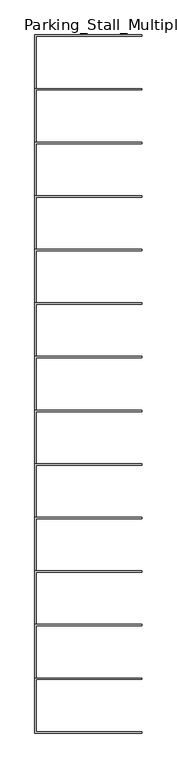
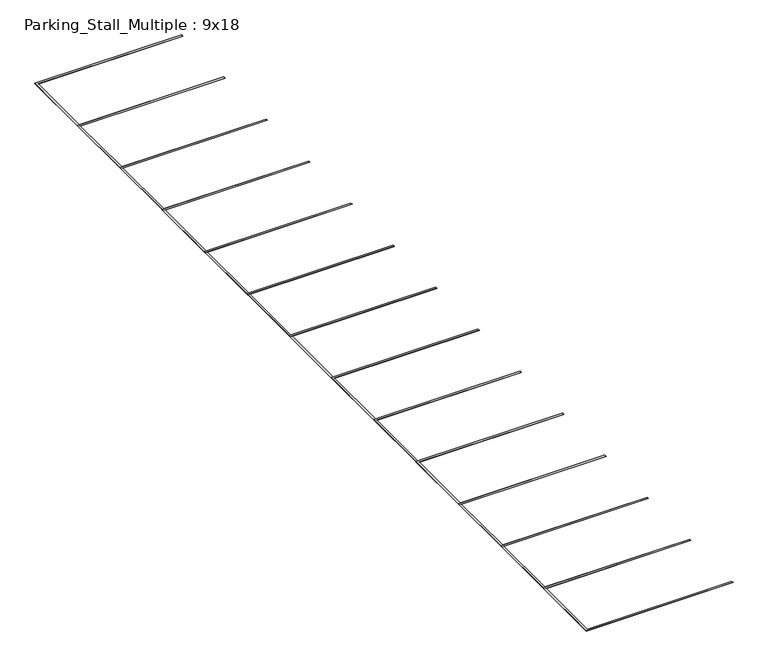
"""IFC4 building model written with IfcOpenShell, lengths in millimetres: proxy geometry, Parking_Stall_Multiple : 9x18."""

from ifc_helpers import new_model, si_unit, origin, origin_with_axes, place, context, project, spatial, polyline, outline, extrude, source, transform, mapped, element, save


def parking_stall_multiple_9x18_eccd42c3(model_context):
    return source(origin(), model_context, "Body", "SweptSolid", [
        extrude(outline(polyline([(5486.4, -32918.4), (5486.4, -32994.6), (76.2, -32994.6), (76.2, -35661.6), (5486.4, -35661.6), (5486.4, -35737.8), (0.0, -35737.8), (0.0, -32918.4), (5486.4, -32918.4)])), origin_with_axes(), (0.0, 0.0, 1.0), 6.35),
        extrude(outline(polyline([(5486.4, -30175.2), (5486.4, -30251.4), (76.2, -30251.4), (76.2, -32918.4), (5486.4, -32918.4), (5486.4, -32994.6), (0.0, -32994.6), (0.0, -30175.2), (5486.4, -30175.2)])), origin_with_axes(), (0.0, 0.0, 1.0), 6.35),
        extrude(outline(polyline([(5486.4, -27432.0), (5486.4, -27508.2), (76.2, -27508.2), (76.2, -30175.2), (5486.4, -30175.2), (5486.4, -30251.4), (0.0, -30251.4), (0.0, -27432.0), (5486.4, -27432.0)])), origin_with_axes(), (0.0, 0.0, 1.0), 6.35),
        extrude(outline(polyline([(5486.4, -24688.8), (5486.4, -24765.0), (76.2, -24765.0), (76.2, -27432.0), (5486.4, -27432.0), (5486.4, -27508.2), (0.0, -27508.2), (0.0, -24688.8), (5486.4, -24688.8)])), origin_with_axes(), (0.0, 0.0, 1.0), 6.35),
        extrude(outline(polyline([(5486.4, -21945.6), (5486.4, -22021.8), (76.2, -22021.8), (76.2, -24688.8), (5486.4, -24688.8), (5486.4, -24765.0), (0.0, -24765.0), (0.0, -21945.6), (5486.4, -21945.6)])), origin_with_axes(), (0.0, 0.0, 1.0), 6.35),
        extrude(outline(polyline([(5486.4, -19202.4), (5486.4, -19278.6), (76.2, -19278.6), (76.2, -21945.6), (5486.4, -21945.6), (5486.4, -22021.8), (0.0, -22021.8), (0.0, -19202.4), (5486.4, -19202.4)])), origin_with_axes(), (0.0, 0.0, 1.0), 6.35),
        extrude(outline(polyline([(5486.4, -16459.2), (5486.4, -16535.4), (76.2, -16535.4), (76.2, -19202.4), (5486.4, -19202.4), (5486.4, -19278.6), (0.0, -19278.6), (0.0, -16459.2), (5486.4, -16459.2)])), origin_with_axes(), (0.0, 0.0, 1.0), 6.35),
        extrude(outline(polyline([(5486.4, -13716.0), (5486.4, -13792.2), (76.2, -13792.2), (76.2, -16459.2), (5486.4, -16459.2), (5486.4, -16535.4), (0.0, -16535.4), (0.0, -13716.0), (5486.4, -13716.0)])), origin_with_axes(), (0.0, 0.0, 1.0), 6.35),
        extrude(outline(polyline([(5486.4, -10972.8), (5486.4, -11049.0), (76.2, -11049.0), (76.2, -13716.0), (5486.4, -13716.0), (5486.4, -13792.2), (0.0, -13792.2), (0.0, -10972.8), (5486.4, -10972.8)])), origin_with_axes(), (0.0, 0.0, 1.0), 6.35),
        extrude(outline(polyline([(5486.4, -8229.6), (5486.4, -8305.8), (76.2, -8305.8), (76.2, -10972.8), (5486.4, -10972.8), (5486.4, -11049.0), (0.0, -11049.0), (0.0, -8229.6), (5486.4, -8229.6)])), origin_with_axes(), (0.0, 0.0, 1.0), 6.35),
        extrude(outline(polyline([(5486.4, -5486.4), (5486.4, -5562.6), (76.2, -5562.6), (76.2, -8229.6), (5486.4, -8229.6), (5486.4, -8305.8), (0.0, -8305.8), (0.0, -5486.4), (5486.4, -5486.4)])), origin_with_axes(), (0.0, 0.0, 1.0), 6.35),
        extrude(outline(polyline([(5486.4, -2743.2), (5486.4, -2819.4), (76.2, -2819.4), (76.2, -5486.4), (5486.4, -5486.4), (5486.4, -5562.6), (0.0, -5562.6), (0.0, -2743.2), (5486.4, -2743.2)])), origin_with_axes(), (0.0, 0.0, 1.0), 6.35),
        extrude(outline(polyline([(5486.4, 0.0), (5486.4, -76.2), (76.2, -76.2), (76.2, -2743.2), (5486.4, -2743.2), (5486.4, -2819.4), (0.0, -2819.4), (0.0, 0.0), (5486.4, 0.0)])), origin_with_axes(), (0.0, 0.0, 1.0), 6.35),
    ])


if __name__ == "__main__":
    model = new_model("IFC4")
    model_context = context("Model", 3, world=origin())
    ifc_project = project(units=[si_unit("LENGTHUNIT", "METRE", prefix="MILLI")], contexts=[model_context])
    site = spatial("IfcSite", under=ifc_project)
    building = spatial("IfcBuilding", under=site)
    placement = place(None, origin())
    parking_stall_multiple_9x18_shape = parking_stall_multiple_9x18_eccd42c3(model_context)
    element("IfcBuildingElementProxy", 1, Name="Parking_Stall_Multiple : 9x18", ObjectType="Parking_Stall_Multiple : 9x18", at=placement, inside=building, context=model_context, shape_type="MappedRepresentation", body=[
        mapped(parking_stall_multiple_9x18_shape, transform((0.0, 0.0, 0.0), x_axis=(1.0, 0.0, 0.0), y_axis=(0.0, 1.0, 0.0), z_axis=(0.0, 0.0, 1.0))),
    ])
    save(model, "model.ifc")

# Revit data of these elements
# Type "Parking_Stall_Multiple : 9x18"
#   Parking_Width_M = 9' - 0"
#   Parking_Run_Length [instance default] = 65' - 0"
#   Parking_Line_Width = 0' - 3"
#   Parking_Length_M = 18' - 0"
#   Single_Parking_Visibility [instance default] = no
#   Parking_ADA_Symbol = no
#   ParkingUnitsArray [instance default] = 7
#   ParkingUnits [instance default] = 7
#   Multiple_Parking_Visibility [instance default] = yes
#   Parking_Line_Material = none
# Element 1 (IfcBuildingElementProxy, "Parking_Stall_Multiple : 9x18")
#   Parking_Run_Length = 115' - 4.25829"
#   ParkingUnitsArray = 13
#   ParkingUnits = 13
